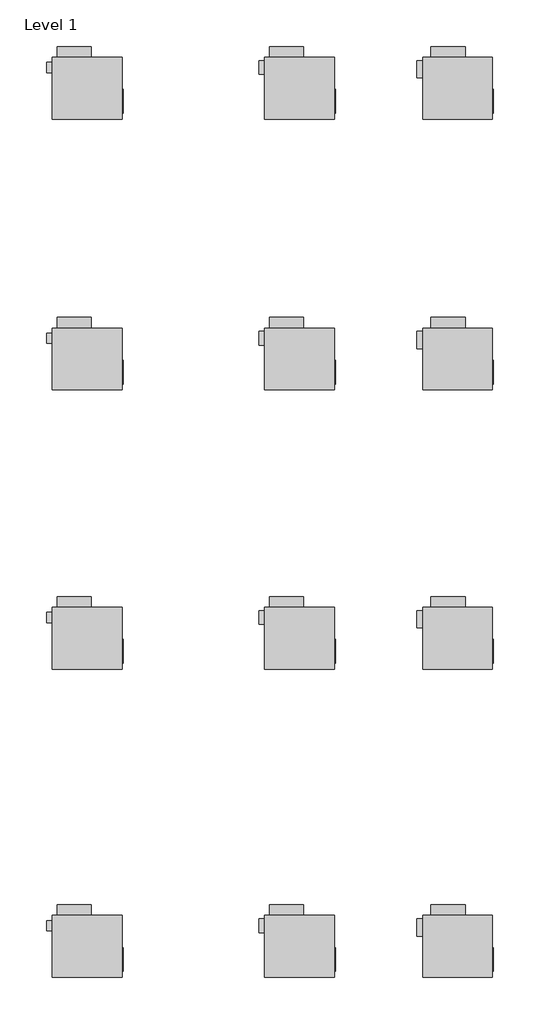
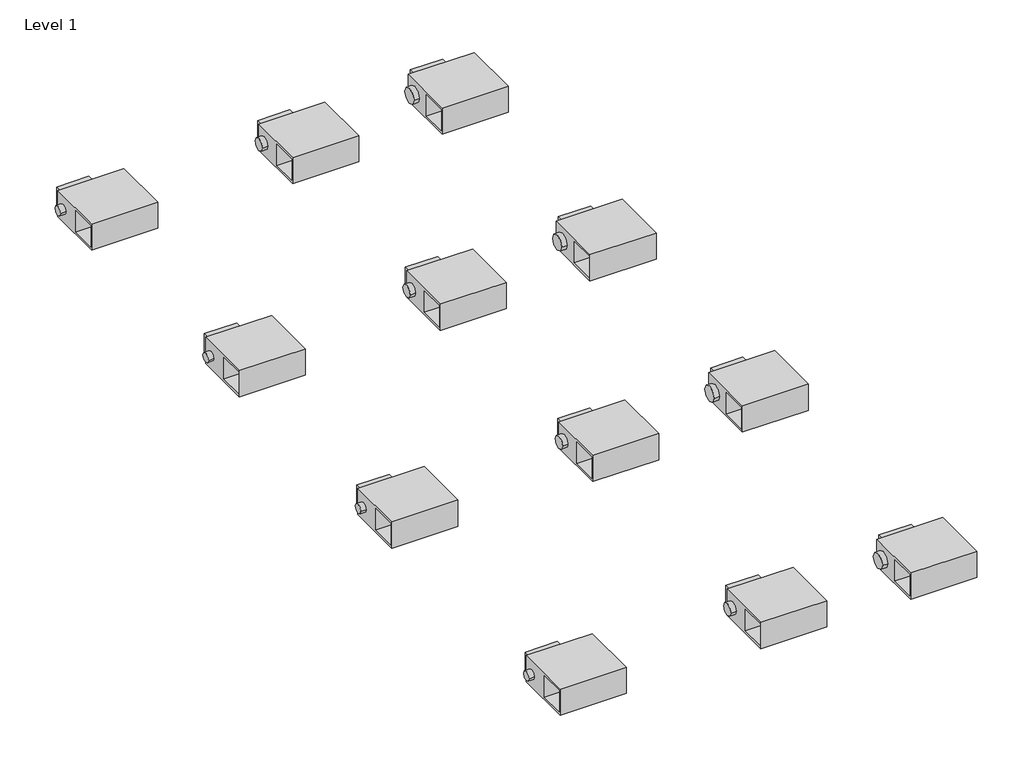
# One storey: 12 proxies.
"""IFC4 building model written with IfcOpenShell, lengths in millimetres."""

import ifcopenshell
import ifcopenshell.guid

model = None  # the IFC model being written
_history = None  # IfcOwnerHistory: only IFC2X3 demands one
_inside = {}  # id of a spatial element -> (the spatial element, [elements in it])
_under = {}  # id of a project, library or spatial element -> (it, [spatial elements below it])
_declared = {}  # id of a project -> (the project, [libraries it declares])
_typed = {}  # id of a type object -> (the type object, [elements of that type])
_made_of = {}  # id of a material, layer set ... -> (it, [elements and type objects made of it])


def new_model(schema):
    """Start an empty IFC model of exactly this schema.

    Asked for "IFC4X3", IfcOpenShell would pick the latest addendum, in which some entities
    have other attributes; the version numbers below select the first issue.
    IFC2X3 requires an IfcOwnerHistory on every rooted entity: one is made here for all.
    """
    global model, _history
    if schema == "IFC4X3":
        model = ifcopenshell.file(schema_version=(4, 3, 0, 0))
    else:
        model = ifcopenshell.file(schema=schema)
    _inside.clear()
    _under.clear()
    _declared.clear()
    _typed.clear()
    _made_of.clear()
    _history = None
    if model.schema == "IFC2X3":
        org = make("IfcOrganization", Name="unknown")
        user = make(
            "IfcPersonAndOrganization",
            ThePerson=make("IfcPerson", FamilyName="unknown"),
            TheOrganization=org,
        )
        app = make(
            "IfcApplication",
            ApplicationDeveloper=org,
            Version="unknown",
            ApplicationFullName="unknown",
            ApplicationIdentifier="unknown",
        )
        _history = make(
            "IfcOwnerHistory",
            OwningUser=user,
            OwningApplication=app,
            ChangeAction="ADDED",
            CreationDate=0,
        )
    return model


def make(cls, **values):
    """One entity of the class cls with the attributes given. An attribute that is None is left unset."""
    return model.create_entity(
        cls, **{name: value for name, value in values.items() if value is not None}
    )


def rooted(cls, **values):
    """An entity with a GlobalId (a new one), such as an element, a storey or a relation."""
    return make(cls, GlobalId=ifcopenshell.guid.new(), OwnerHistory=_history, **values)


def si_unit(unit_type, name, prefix=None):
    """IfcSIUnit, for example si_unit("LENGTHUNIT", "METRE", prefix="MILLI")."""
    return make("IfcSIUnit", UnitType=unit_type, Prefix=prefix, Name=name)


def assignment(units):
    """IfcUnitAssignment: the units of a project."""
    return None if units is None else make("IfcUnitAssignment", Units=units)


def point(xyz):
    """IfcCartesianPoint."""
    return None if xyz is None else make("IfcCartesianPoint", Coordinates=xyz)


def direction(xyz):
    """IfcDirection."""
    return None if xyz is None else make("IfcDirection", DirectionRatios=xyz)


def frame(location, z_axis=None, x_axis=None):
    """IfcAxis2Placement3D, a coordinate frame: its origin and axes. An axis left out is left unset."""
    return make(
        "IfcAxis2Placement3D",
        Location=point(location),
        Axis=direction(z_axis),
        RefDirection=direction(x_axis),
    )


def frame_2d(location, x_axis=None):
    """IfcAxis2Placement2D, a coordinate frame in the plane: its origin and x axis."""
    return make(
        "IfcAxis2Placement2D", Location=point(location), RefDirection=direction(x_axis)
    )


def origin():
    """The frame at (0, 0, 0) with its axes left unset."""
    return frame((0.0, 0.0, 0.0))


def place(relative_to, where):
    """IfcLocalPlacement: puts the frame where relative to a parent placement (None: the world)."""
    return make(
        "IfcLocalPlacement", PlacementRelTo=relative_to, RelativePlacement=where
    )


def context(
    kind, dimensions, precision=None, world=None, true_north=None, identifier=None
):
    """IfcGeometricRepresentationContext, for example the 3D "Model" context."""
    return make(
        "IfcGeometricRepresentationContext",
        ContextIdentifier=identifier,
        ContextType=kind,
        CoordinateSpaceDimension=dimensions,
        Precision=precision,
        WorldCoordinateSystem=world,
        TrueNorth=true_north,
    )


def project(units=None, contexts=None):
    """IfcProject with its units and contexts."""
    return rooted(
        "IfcProject",
        Name="project",
        RepresentationContexts=contexts,
        UnitsInContext=assignment(units),
    )


def spatial(cls, under=None, at=None, **own):
    """A site, building, storey or space (cls), placed at a placement, below another one or the project."""
    s = rooted(cls, ObjectPlacement=at, **own)
    if under is not None:
        _under.setdefault(under.id(), (under, []))[1].append(s)
    return s


def polyline(points):
    """IfcPolyline through the points."""
    return make("IfcPolyline", Points=[point(p) for p in points])


def circle_curve(where, radius):
    """IfcCircle in the frame where."""
    return make("IfcCircle", Position=where, Radius=radius)


def trimmed(basis, trim1, trim2, sense, master):
    """IfcTrimmedCurve: the piece of a basis curve between two trims."""
    return make(
        "IfcTrimmedCurve",
        BasisCurve=basis,
        Trim1=trim1,
        Trim2=trim2,
        SenseAgreement=sense,
        MasterRepresentation=master,
    )


def segment(curve, same_sense, transition):
    """IfcCompositeCurveSegment."""
    return make(
        "IfcCompositeCurveSegment",
        Transition=transition,
        SameSense=same_sense,
        ParentCurve=curve,
    )


def composite_curve(segments, self_intersect=None):
    """IfcCompositeCurve: segments joined end to end."""
    return make("IfcCompositeCurve", Segments=segments, SelfIntersect=self_intersect)


def outline(outer, holes=None, kind="AREA"):
    """IfcArbitraryClosedProfileDef: a profile drawn as a closed curve; with holes, ...WithVoids."""
    if holes is None:
        return make("IfcArbitraryClosedProfileDef", ProfileType=kind, OuterCurve=outer)
    return make(
        "IfcArbitraryProfileDefWithVoids",
        ProfileType=kind,
        OuterCurve=outer,
        InnerCurves=holes,
    )


def extrude(swept, where, along, depth):
    """IfcExtrudedAreaSolid: the profile swept, set in the frame where, extruded along a direction by depth."""
    return make(
        "IfcExtrudedAreaSolid",
        SweptArea=swept,
        Position=where,
        ExtrudedDirection=direction(along),
        Depth=depth,
    )


def faces_of(points, faces, orient=None, outer=None):
    """IfcFace entities. A face is a list of loops; a loop is a list of indices into points, from 0.

    orient and outer hold one flag for each loop. By default every Orientation is true, the
    first loop of a face is its IfcFaceOuterBound and the others are IfcFaceBound.
    """
    made = []
    for i, loops in enumerate(faces):
        bounds = []
        for j, loop in enumerate(loops):
            is_outer = j == 0 if outer is None else outer[i][j]
            bounds.append(
                make(
                    "IfcFaceOuterBound" if is_outer else "IfcFaceBound",
                    Bound=make("IfcPolyLoop", Polygon=[points[k] for k in loop]),
                    Orientation=True if orient is None else orient[i][j],
                )
            )
        made.append(make("IfcFace", Bounds=bounds))
    return made


def faceted_brep(points, faces, orient=None, outer=None, voids=None):
    """IfcFacetedBrep: a solid bounded by flat faces; with voids (closed shells), ...WithVoids."""
    shared = [point(p) for p in points]
    hull = make("IfcClosedShell", CfsFaces=faces_of(shared, faces, orient, outer))
    if voids is None:
        return make("IfcFacetedBrep", Outer=hull)
    return make(
        "IfcFacetedBrepWithVoids",
        Outer=hull,
        Voids=[
            make(cls, CfsFaces=faces_of(shared, fs, o, b)) for cls, fs, o, b in voids
        ],
    )


def shape(context_of_items, identifier, shape_type, items):
    """IfcShapeRepresentation: the items that make up one representation, for example the "Body"."""
    return make(
        "IfcShapeRepresentation",
        ContextOfItems=context_of_items,
        RepresentationIdentifier=identifier,
        RepresentationType=shape_type,
        Items=items,
    )


def source(mapping_origin, context_of_items, identifier, shape_type, items):
    """IfcRepresentationMap: a shape defined once, which mapped items show again and again."""
    return make(
        "IfcRepresentationMap",
        MappingOrigin=mapping_origin,
        MappedRepresentation=shape(context_of_items, identifier, shape_type, items),
    )


def transform(
    local_origin,
    x_axis=None,
    y_axis=None,
    z_axis=None,
    scale=None,
    scale2=None,
    scale3=None,
    uniform=True,
):
    """IfcCartesianTransformationOperator3D, or its non-uniform kind. x_axis, y_axis, z_axis: its Axis1, 2, 3."""
    if uniform:
        return make(
            "IfcCartesianTransformationOperator3D",
            Axis1=direction(x_axis),
            Axis2=direction(y_axis),
            LocalOrigin=point(local_origin),
            Scale=scale,
            Axis3=direction(z_axis),
        )
    return make(
        "IfcCartesianTransformationOperator3DnonUniform",
        Axis1=direction(x_axis),
        Axis2=direction(y_axis),
        LocalOrigin=point(local_origin),
        Scale=scale,
        Axis3=direction(z_axis),
        Scale2=scale2,
        Scale3=scale3,
    )


def mapped(mapping_source, mapping_target):
    """IfcMappedItem: shows the shape of a source again, moved by a transform."""
    return make(
        "IfcMappedItem", MappingSource=mapping_source, MappingTarget=mapping_target
    )


def made_of(thing, what):
    """Note that an element or type object is made of a material, layer set ...; save() writes the relation."""
    if what is not None:
        _made_of.setdefault(what.id(), (what, []))[1].append(thing)
    return thing


def element(
    cls,
    number,
    at=None,
    inside=None,
    cuts=None,
    type_object=None,
    material=None,
    context=None,
    identifier="Body",
    shape_type=None,
    held_by="IfcProductDefinitionShape",
    body=None,
    shapes=None,
    **own,
):
    """One element of the class cls, such as IfcWall. Its Tag is "e" and its number.

    at: its placement. inside: the storey or other place that contains it. cuts: it is an
    opening in that element (IfcRelVoidsElement). A single representation is given by context,
    identifier, shape_type and body (its items); several are given by shapes. held_by: the class
    of the entity that holds the representations. save() writes the other relations.
    """
    e = rooted(cls, Tag="e%d" % number, ObjectPlacement=at, **own)
    if body is not None:
        shapes = [shape(context, identifier, shape_type, body)]
    if shapes is not None:
        e.Representation = make(held_by, Representations=shapes)
    if inside is not None:
        _inside.setdefault(inside.id(), (inside, []))[1].append(e)
    if cuts is not None:
        rooted(
            "IfcRelVoidsElement", RelatingBuildingElement=cuts, RelatedOpeningElement=e
        )
    if type_object is not None:
        _typed.setdefault(type_object.id(), (type_object, []))[1].append(e)
    return made_of(e, material)


def aggregate(whole, parts):
    """IfcRelAggregates: a whole, such as a stair, and the parts it consists of."""
    return rooted("IfcRelAggregates", RelatingObject=whole, RelatedObjects=parts)


def save(model, path):
    """Write the relations noted so far, then the file.

    IfcRelAggregates (storeys below a building ...), IfcRelContainedInSpatialStructure (elements
    in a storey), IfcRelDefinesByType, IfcRelAssociatesMaterial and IfcRelDeclares: one each for
    every whole, place, type object, material and project.
    """
    for whole, parts in _under.values():
        aggregate(whole, parts)
    for where, things in _inside.values():
        rooted(
            "IfcRelContainedInSpatialStructure",
            RelatedElements=things,
            RelatingStructure=where,
        )
    for kind, things in _typed.values():
        rooted("IfcRelDefinesByType", RelatedObjects=things, RelatingType=kind)
    for what, things in _made_of.values():
        rooted("IfcRelAssociatesMaterial", RelatedObjects=things, RelatingMaterial=what)
    for by, libraries in _declared.values():
        rooted("IfcRelDeclares", RelatingContext=by, RelatedDefinitions=libraries)
    model.write(path)


def vav_unit_parallel_fan_powered_size_2_10_inch_inlet_b65b1531(model_context):
    return source(origin(), model_context, "Body", "SolidModel", [
        extrude(outline(polyline([(531.8125, -15.875), (531.8125, -371.475), (519.1125, -371.475), (519.1125, -15.875), (531.8125, -15.875)])), frame((0.0, 0.0, -139.7), z_axis=(0.0, 0.0, 1.0), x_axis=(1.0, 0.0, 0.0)), (0.0, 0.0, 1.0), 279.4),
        extrude(outline(polyline([(112.7125, 460.375), (-395.2875, 460.375), (-395.2875, 619.125), (112.7125, 619.125), (112.7125, 460.375)])), frame((0.0, 0.0, -152.4), z_axis=(0.0, 0.0, 1.0), x_axis=(1.0, 0.0, 0.0)), (0.0, 0.0, 1.0), 304.8),
        extrude(outline(composite_curve([segment(trimmed(circle_curve(frame_2d((282.575, 0.0)), 127.0), [point((155.575, 0.0))], [point((409.575, 0.0))], False, "CARTESIAN"), True, "CONTINUOUS"), segment(trimmed(circle_curve(frame_2d((282.575, 0.0)), 127.0), [point((409.575, 0.0))], [point((155.575, 0.0))], False, "CARTESIAN"), True, "CONTINUOUS")], self_intersect=False)), frame((-604.8375, 0.0, 0.0), z_axis=(1.0, 0.0, 0.0), x_axis=(0.0, 1.0, 0.0)), (0.0, 0.0, 1.0), 85.725),
        faceted_brep([(519.1125, 460.375, 217.4875), (-519.1125, 460.375, 217.4875), (-519.1125, -460.375, 217.4875), (519.1125, -460.375, 217.4875), (519.1125, 460.375, -217.4875), (519.1125, -460.375, -217.4875), (-519.1125, -460.375, -217.4875), (-519.1125, 460.375, -217.4875), (-519.1125, -434.975, 177.8), (-519.1125, -434.975, -177.8), (-519.1125, -28.575, -177.8), (-519.1125, -28.575, 177.8), (0.0, -434.975, 177.8), (0.0, -28.575, 177.8), (0.0, -28.575, -177.8), (0.0, -434.975, -177.8)], [[[0, 1, 2, 3]], [[4, 5, 6, 7]], [[1, 0, 4, 7]], [[2, 1, 7, 6], [8, 9, 10, 11]], [[3, 2, 6, 5]], [[0, 3, 5, 4]], [[12, 13, 14, 15]], [[12, 15, 9, 8]], [[15, 14, 10, 9]], [[14, 13, 11, 10]], [[13, 12, 8, 11]]]),
    ])


def vav_unit_parallel_fan_powered_size_2_6_inch_inlet_6222e6d5(model_context):
    return source(origin(), model_context, "Body", "SolidModel", [
        extrude(outline(polyline([(531.8125, -15.875), (531.8125, -371.475), (519.1125, -371.475), (519.1125, -15.875), (531.8125, -15.875)])), frame((0.0, 0.0, -139.7), z_axis=(0.0, 0.0, 1.0), x_axis=(1.0, 0.0, 0.0)), (0.0, 0.0, 1.0), 279.4),
        extrude(outline(polyline([(61.9125, 460.375), (-446.0875, 460.375), (-446.0875, 619.125), (61.9125, 619.125), (61.9125, 460.375)])), frame((0.0, 0.0, -152.4), z_axis=(0.0, 0.0, 1.0), x_axis=(1.0, 0.0, 0.0)), (0.0, 0.0, 1.0), 304.8),
        extrude(outline(composite_curve([segment(trimmed(circle_curve(frame_2d((307.975, 0.0)), 76.2), [point((231.775, 0.0))], [point((384.175, 0.0))], False, "CARTESIAN"), True, "CONTINUOUS"), segment(trimmed(circle_curve(frame_2d((307.975, 0.0)), 76.2), [point((384.175, 0.0))], [point((231.775, 0.0))], False, "CARTESIAN"), True, "CONTINUOUS")], self_intersect=False)), frame((-604.8375, 0.0, 0.0), z_axis=(1.0, 0.0, 0.0), x_axis=(0.0, 1.0, 0.0)), (0.0, 0.0, 1.0), 85.725),
        faceted_brep([(519.1125, 460.375, 217.4875), (-519.1125, 460.375, 217.4875), (-519.1125, -460.375, 217.4875), (519.1125, -460.375, 217.4875), (519.1125, 460.375, -217.4875), (519.1125, -460.375, -217.4875), (-519.1125, -460.375, -217.4875), (-519.1125, 460.375, -217.4875), (-519.1125, -434.975, 177.8), (-519.1125, -434.975, -177.8), (-519.1125, -28.575, -177.8), (-519.1125, -28.575, 177.8), (0.0, -434.975, 177.8), (0.0, -28.575, 177.8), (0.0, -28.575, -177.8), (0.0, -434.975, -177.8)], [[[0, 1, 2, 3]], [[4, 5, 6, 7]], [[1, 0, 4, 7]], [[2, 1, 7, 6], [8, 9, 10, 11]], [[3, 2, 6, 5]], [[0, 3, 5, 4]], [[12, 13, 14, 15]], [[12, 15, 9, 8]], [[15, 14, 10, 9]], [[14, 13, 11, 10]], [[13, 12, 8, 11]]]),
    ])


def vav_unit_parallel_fan_powered_size_2_8_inch_inlet_1779b90c(model_context):
    return source(origin(), model_context, "Body", "SolidModel", [
        extrude(outline(polyline([(531.8125, -15.875), (531.8125, -371.475), (519.1125, -371.475), (519.1125, -15.875), (531.8125, -15.875)])), frame((0.0, 0.0, -139.7), z_axis=(0.0, 0.0, 1.0), x_axis=(1.0, 0.0, 0.0)), (0.0, 0.0, 1.0), 279.4),
        extrude(outline(polyline([(61.9125, 460.375), (-446.0875, 460.375), (-446.0875, 619.125), (61.9125, 619.125), (61.9125, 460.375)])), frame((0.0, 0.0, -152.4), z_axis=(0.0, 0.0, 1.0), x_axis=(1.0, 0.0, 0.0)), (0.0, 0.0, 1.0), 304.8),
        extrude(outline(composite_curve([segment(trimmed(circle_curve(frame_2d((307.975, 0.0)), 101.6), [point((206.375, 0.0))], [point((409.575, 0.0))], False, "CARTESIAN"), True, "CONTINUOUS"), segment(trimmed(circle_curve(frame_2d((307.975, 0.0)), 101.6), [point((409.575, 0.0))], [point((206.375, 0.0))], False, "CARTESIAN"), True, "CONTINUOUS")], self_intersect=False)), frame((-604.8375, 0.0, 0.0), z_axis=(1.0, 0.0, 0.0), x_axis=(0.0, 1.0, 0.0)), (0.0, 0.0, 1.0), 85.725),
        faceted_brep([(519.1125, 460.375, 217.4875), (-519.1125, 460.375, 217.4875), (-519.1125, -460.375, 217.4875), (519.1125, -460.375, 217.4875), (519.1125, 460.375, -217.4875), (519.1125, -460.375, -217.4875), (-519.1125, -460.375, -217.4875), (-519.1125, 460.375, -217.4875), (-519.1125, -434.975, 177.8), (-519.1125, -434.975, -177.8), (-519.1125, -28.575, -177.8), (-519.1125, -28.575, 177.8), (0.0, -434.975, 177.8), (0.0, -28.575, 177.8), (0.0, -28.575, -177.8), (0.0, -434.975, -177.8)], [[[0, 1, 2, 3]], [[4, 5, 6, 7]], [[1, 0, 4, 7]], [[2, 1, 7, 6], [8, 9, 10, 11]], [[3, 2, 6, 5]], [[0, 3, 5, 4]], [[12, 13, 14, 15]], [[12, 15, 9, 8]], [[15, 14, 10, 9]], [[14, 13, 11, 10]], [[13, 12, 8, 11]]]),
    ])


model = new_model("IFC4")

# Units and contexts
model_context = context("Model", 3, world=origin())
ifc_project = project(units=[si_unit("LENGTHUNIT", "METRE", prefix="MILLI")], contexts=[model_context])

# Site, building, storey
site = spatial("IfcSite", under=ifc_project)
building = spatial("IfcBuilding", under=site)
storey = spatial("IfcBuildingStorey", under=building, Name="Level 1", Elevation=0.0)

# Proxies
placement = place(None, origin())
vav_unit_parallel_fan_powered_size_2_10_inch_inlet_shape = vav_unit_parallel_fan_powered_size_2_10_inch_inlet_b65b1531(model_context)
element("IfcBuildingElementProxy", 1, Name="VAV Unit - Parallel Fan Powered : Size 2 - 10 inch Inlet", ObjectType="VAV Unit - Parallel Fan Powered : Size 2 - 10 inch Inlet", at=placement, inside=storey, context=model_context, shape_type="MappedRepresentation", body=[
    mapped(vav_unit_parallel_fan_powered_size_2_10_inch_inlet_shape, transform((-7137.4442191, 12797.9424061, 0.0), x_axis=(1.0, 0.0, 0.0), y_axis=(0.0, 1.0, 0.0), z_axis=(0.0, 0.0, 1.0))),
])
element("IfcBuildingElementProxy", 2, Name="VAV Unit - Parallel Fan Powered : Size 2 - 10 inch Inlet", ObjectType="VAV Unit - Parallel Fan Powered : Size 2 - 10 inch Inlet", at=placement, inside=storey, context=model_context, shape_type="MappedRepresentation", body=[
    mapped(vav_unit_parallel_fan_powered_size_2_10_inch_inlet_shape, transform((-7137.4442191, 8773.2773935, 0.0), x_axis=(1.0, 0.0, 0.0), y_axis=(0.0, 1.0, 0.0), z_axis=(0.0, 0.0, 1.0))),
])
element("IfcBuildingElementProxy", 3, Name="VAV Unit - Parallel Fan Powered : Size 2 - 10 inch Inlet", ObjectType="VAV Unit - Parallel Fan Powered : Size 2 - 10 inch Inlet", at=placement, inside=storey, context=model_context, shape_type="MappedRepresentation", body=[
    mapped(vav_unit_parallel_fan_powered_size_2_10_inch_inlet_shape, transform((-7137.4442191, 4624.7765344, 0.0), x_axis=(1.0, 0.0, 0.0), y_axis=(0.0, 1.0, 0.0), z_axis=(0.0, 0.0, 1.0))),
])
element("IfcBuildingElementProxy", 4, Name="VAV Unit - Parallel Fan Powered : Size 2 - 10 inch Inlet", ObjectType="VAV Unit - Parallel Fan Powered : Size 2 - 10 inch Inlet", at=placement, inside=storey, context=model_context, shape_type="MappedRepresentation", body=[
    mapped(vav_unit_parallel_fan_powered_size_2_10_inch_inlet_shape, transform((-7137.4442191, 42.8502123, 0.0), x_axis=(1.0, 0.0, 0.0), y_axis=(0.0, 1.0, 0.0), z_axis=(0.0, 0.0, 1.0))),
])
vav_unit_parallel_fan_powered_size_2_6_inch_inlet_shape = vav_unit_parallel_fan_powered_size_2_6_inch_inlet_6222e6d5(model_context)
element("IfcBuildingElementProxy", 5, Name="VAV Unit - Parallel Fan Powered : Size 2 - 6 inch Inlet", ObjectType="VAV Unit - Parallel Fan Powered : Size 2 - 6 inch Inlet", at=placement, inside=storey, context=model_context, shape_type="MappedRepresentation", body=[
    mapped(vav_unit_parallel_fan_powered_size_2_6_inch_inlet_shape, transform((-12648.1393902, 12797.9424061, 0.0), x_axis=(1.0, 0.0, 0.0), y_axis=(0.0, 1.0, 0.0), z_axis=(0.0, 0.0, 1.0))),
])
element("IfcBuildingElementProxy", 6, Name="VAV Unit - Parallel Fan Powered : Size 2 - 6 inch Inlet", ObjectType="VAV Unit - Parallel Fan Powered : Size 2 - 6 inch Inlet", at=placement, inside=storey, context=model_context, shape_type="MappedRepresentation", body=[
    mapped(vav_unit_parallel_fan_powered_size_2_6_inch_inlet_shape, transform((-12648.1393902, 8773.2773935, 0.0), x_axis=(1.0, 0.0, 0.0), y_axis=(0.0, 1.0, 0.0), z_axis=(0.0, 0.0, 1.0))),
])
element("IfcBuildingElementProxy", 7, Name="VAV Unit - Parallel Fan Powered : Size 2 - 6 inch Inlet", ObjectType="VAV Unit - Parallel Fan Powered : Size 2 - 6 inch Inlet", at=placement, inside=storey, context=model_context, shape_type="MappedRepresentation", body=[
    mapped(vav_unit_parallel_fan_powered_size_2_6_inch_inlet_shape, transform((-12648.1393902, 4624.7765344, 0.0), x_axis=(1.0, 0.0, 0.0), y_axis=(0.0, 1.0, 0.0), z_axis=(0.0, 0.0, 1.0))),
])
element("IfcBuildingElementProxy", 8, Name="VAV Unit - Parallel Fan Powered : Size 2 - 6 inch Inlet", ObjectType="VAV Unit - Parallel Fan Powered : Size 2 - 6 inch Inlet", at=placement, inside=storey, context=model_context, shape_type="MappedRepresentation", body=[
    mapped(vav_unit_parallel_fan_powered_size_2_6_inch_inlet_shape, transform((-12648.1393902, 42.8502123, 0.0), x_axis=(1.0, 0.0, 0.0), y_axis=(0.0, 1.0, 0.0), z_axis=(0.0, 0.0, 1.0))),
])
vav_unit_parallel_fan_powered_size_2_8_inch_inlet_shape = vav_unit_parallel_fan_powered_size_2_8_inch_inlet_1779b90c(model_context)
element("IfcBuildingElementProxy", 9, Name="VAV Unit - Parallel Fan Powered : Size 2 - 8 inch Inlet", ObjectType="VAV Unit - Parallel Fan Powered : Size 2 - 8 inch Inlet", at=placement, inside=storey, context=model_context, shape_type="MappedRepresentation", body=[
    mapped(vav_unit_parallel_fan_powered_size_2_8_inch_inlet_shape, transform((-9490.3253034, 12797.9424061, 0.0), x_axis=(1.0, 0.0, 0.0), y_axis=(0.0, 1.0, 0.0), z_axis=(0.0, 0.0, 1.0))),
])
element("IfcBuildingElementProxy", 10, Name="VAV Unit - Parallel Fan Powered : Size 2 - 8 inch Inlet", ObjectType="VAV Unit - Parallel Fan Powered : Size 2 - 8 inch Inlet", at=placement, inside=storey, context=model_context, shape_type="MappedRepresentation", body=[
    mapped(vav_unit_parallel_fan_powered_size_2_8_inch_inlet_shape, transform((-9490.3253034, 8773.2773935, 0.0), x_axis=(1.0, 0.0, 0.0), y_axis=(0.0, 1.0, 0.0), z_axis=(0.0, 0.0, 1.0))),
])
element("IfcBuildingElementProxy", 11, Name="VAV Unit - Parallel Fan Powered : Size 2 - 8 inch Inlet", ObjectType="VAV Unit - Parallel Fan Powered : Size 2 - 8 inch Inlet", at=placement, inside=storey, context=model_context, shape_type="MappedRepresentation", body=[
    mapped(vav_unit_parallel_fan_powered_size_2_8_inch_inlet_shape, transform((-9490.3253034, 4624.7765344, 0.0), x_axis=(1.0, 0.0, 0.0), y_axis=(0.0, 1.0, 0.0), z_axis=(0.0, 0.0, 1.0))),
])
element("IfcBuildingElementProxy", 12, Name="VAV Unit - Parallel Fan Powered : Size 2 - 8 inch Inlet", ObjectType="VAV Unit - Parallel Fan Powered : Size 2 - 8 inch Inlet", at=placement, inside=storey, context=model_context, shape_type="MappedRepresentation", body=[
    mapped(vav_unit_parallel_fan_powered_size_2_8_inch_inlet_shape, transform((-9490.3253034, 42.8502123, 0.0), x_axis=(1.0, 0.0, 0.0), y_axis=(0.0, 1.0, 0.0), z_axis=(0.0, 0.0, 1.0))),
])

save(model, "model.ifc")

# Revit data of these elements
# Project information
#   Project Issue Date = "Issue Date"
#   Project Status = "Project Status"
#   Client Name = "Owner"
#   Project Address = "Enter address here"
#   Project Name = "Project Name"
#   Project Number = "Project Number"
# Type "VAV Unit - Parallel Fan Powered : Size 2 - 10 inch Inlet"
#   Width2 = 1' - 2"
#   Voltage = 120 V
#   UnitWidth = 3' - 4 7/8"
#   UnitHeight = 3' - 0 1/4"
#   UnitDepth = 1' - 5 1/8"
#   SupplyConnectorWidth = 1' - 2"
#   SupplyConnectorVerticalOffset = 0' - 2 1/8"
#   SupplyConnectorLength = 0' - 0 1/2"
#   SupplyConnectorHorizontalOffset = 0' - 3 1/2"
#   SupplyConnectorDepth = 0' - 11"
#   SupplyAirConnectorCenterOffset = 0' - 10 1/2"
#   PrimaryToSupplyRatio [instance default] = 0.2
#   PrimaryAirOffset = 0' - 7"
#   PrimaryAirFlow [instance default] = 280 CFM
#   PrimaryAirConnectorVerticalOffset = 0' - 8 9/16"
#   PrimaryAirConnectorRadius = 0' - 5"
#   PrimaryAirConnectorLength = 0' - 3 3/8"
#   PrimaryAirConnectorDiameter = 0' - 10"
#   PrimaryAirConnectorCenterOffset = 0' - 7"
#   Pressure Drop [instance default] = 0.01 in-wg
#   InducedAirInletWidth = 1' - 4"
#   InducedAirInletDepth = 1' - 2"
#   InducedAirConnectorHorizontalOffset = 0' - 1"
#   InducedAirConnectorCenterOffset = 0' - 9"
#   Height2 = 0' - 11"
#   ElectricalConnectionBoxWidth = 1' - 8"
#   ElectricalConnectionBoxOffset = 0' - 4 7/8"
#   ElectricalConnectionBoxHeight = 0' - 6 1/4"
#   ElectricalConnectionBoxDepth = 1' - 0"
#   SupplyAirFlow [instance default] = 1400 CFM
#   Apparent Load = 542 VA
#   SupplyAirConnectorIndex = 2
#   PrimaryAirConnectorIndex = 1
#   Number of Poles = 1
#   InducedAirConnectorIndex = 3
#   VAV Material = none
#   Load Classification = Cooling
#   Default Elevation = 0
#   Assembly Code = ""
# Type "VAV Unit - Parallel Fan Powered : Size 2 - 6 inch Inlet"
#   Width2 = 1' - 2"
#   Voltage = 120 V
#   UnitWidth = 3' - 4 7/8"
#   UnitHeight = 3' - 0 1/4"
#   UnitDepth = 1' - 5 1/8"
#   SupplyConnectorWidth = 1' - 2"
#   SupplyConnectorVerticalOffset = 0' - 2 1/8"
#   SupplyConnectorLength = 0' - 0 1/2"
#   SupplyConnectorHorizontalOffset = 0' - 3 1/2"
#   SupplyConnectorDepth = 0' - 11"
#   SupplyAirConnectorCenterOffset = 0' - 10 1/2"
#   PrimaryToSupplyRatio [instance default] = 0.2
#   PrimaryAirOffset = 0' - 6"
#   PrimaryAirFlow [instance default] = 100 CFM
#   PrimaryAirConnectorVerticalOffset = 0' - 8 9/16"
#   PrimaryAirConnectorRadius = 0' - 3"
#   PrimaryAirConnectorLength = 0' - 3 3/8"
#   PrimaryAirConnectorDiameter = 0' - 6"
#   PrimaryAirConnectorCenterOffset = 0' - 6"
#   Pressure Drop [instance default] = 0.04 in-wg
#   InducedAirInletWidth = 1' - 4"
#   InducedAirInletDepth = 1' - 2"
#   InducedAirConnectorHorizontalOffset = 0' - 1"
#   InducedAirConnectorCenterOffset = 0' - 9"
#   Height2 = 0' - 11"
#   ElectricalConnectionBoxWidth = 1' - 8"
#   ElectricalConnectionBoxOffset = 0' - 2 7/8"
#   ElectricalConnectionBoxHeight = 0' - 6 1/4"
#   ElectricalConnectionBoxDepth = 1' - 0"
#   SupplyAirFlow [instance default] = 500 CFM
#   Apparent Load = 181 VA
#   SupplyAirConnectorIndex = 2
#   PrimaryAirConnectorIndex = 1
#   Number of Poles = 1
#   InducedAirConnectorIndex = 3
#   VAV Material = none
#   Load Classification = Cooling
#   Default Elevation = 0
#   Assembly Code = ""
# Type "VAV Unit - Parallel Fan Powered : Size 2 - 8 inch Inlet"
#   Width2 = 1' - 2"
#   Voltage = 120 V
#   UnitWidth = 3' - 4 7/8"
#   UnitHeight = 3' - 0 1/4"
#   UnitDepth = 1' - 5 1/8"
#   SupplyConnectorWidth = 1' - 2"
#   SupplyConnectorVerticalOffset = 0' - 2 1/8"
#   SupplyConnectorLength = 0' - 0 1/2"
#   SupplyConnectorHorizontalOffset = 0' - 3 1/2"
#   SupplyConnectorDepth = 0' - 11"
#   SupplyAirConnectorCenterOffset = 0' - 10 1/2"
#   PrimaryToSupplyRatio [instance default] = 0.2
#   PrimaryAirOffset = 0' - 6"
#   PrimaryAirFlow [instance default] = 180 CFM
#   PrimaryAirConnectorVerticalOffset = 0' - 8 9/16"
#   PrimaryAirConnectorRadius = 0' - 4"
#   PrimaryAirConnectorLength = 0' - 3 3/8"
#   PrimaryAirConnectorDiameter = 0' - 8"
#   PrimaryAirConnectorCenterOffset = 0' - 6"
#   Pressure Drop [instance default] = 0.02 in-wg
#   InducedAirInletWidth = 1' - 4"
#   InducedAirInletDepth = 1' - 2"
#   InducedAirConnectorHorizontalOffset = 0' - 1"
#   InducedAirConnectorCenterOffset = 0' - 9"
#   Height2 = 0' - 11"
#   ElectricalConnectionBoxWidth = 1' - 8"
#   ElectricalConnectionBoxOffset = 0' - 2 7/8"
#   ElectricalConnectionBoxHeight = 0' - 6 1/4"
#   ElectricalConnectionBoxDepth = 1' - 0"
#   SupplyAirFlow [instance default] = 900 CFM
#   Apparent Load = 271 VA
#   SupplyAirConnectorIndex = 2
#   PrimaryAirConnectorIndex = 1
#   Number of Poles = 1
#   InducedAirConnectorIndex = 3
#   VAV Material = none
#   Load Classification = Cooling
#   Default Elevation = 0
#   Assembly Code = ""
# Element 1 (IfcBuildingElementProxy, "VAV Unit - Parallel Fan Powered : Size 2 - 10 inch Inlet")
#   Mark = "9"
#   SupplyAirFlow = 1400 CFM
#   PrimaryToSupplyRatio = 0.2
#   PrimaryAirFlow = 280 CFM
#   Pressure Drop = 0.01 in-wg
#   Phase Created = New Construction
# Element 2 (IfcBuildingElementProxy, "VAV Unit - Parallel Fan Powered : Size 2 - 10 inch Inlet")
#   Mark = "10"
#   SupplyAirFlow = 1400 CFM
#   PrimaryToSupplyRatio = 0.2
#   PrimaryAirFlow = 280 CFM
#   Pressure Drop = 0.01 in-wg
#   Phase Created = New Construction
# Element 3 (IfcBuildingElementProxy, "VAV Unit - Parallel Fan Powered : Size 2 - 10 inch Inlet")
#   Mark = "11"
#   SupplyAirFlow = 1400 CFM
#   PrimaryToSupplyRatio = 0.2
#   PrimaryAirFlow = 280 CFM
#   Pressure Drop = 0.01 in-wg
#   Phase Created = New Construction
# Element 4 (IfcBuildingElementProxy, "VAV Unit - Parallel Fan Powered : Size 2 - 10 inch Inlet")
#   Mark = "12"
#   SupplyAirFlow = 1400 CFM
#   PrimaryToSupplyRatio = 0.2
#   PrimaryAirFlow = 280 CFM
#   Pressure Drop = 0.01 in-wg
#   Phase Created = New Construction
# Element 5 (IfcBuildingElementProxy, "VAV Unit - Parallel Fan Powered : Size 2 - 6 inch Inlet")
#   Mark = "1"
#   SupplyAirFlow = 500 CFM
#   PrimaryToSupplyRatio = 0.2
#   PrimaryAirFlow = 100 CFM
#   Pressure Drop = 0.04 in-wg
#   Phase Created = New Construction
# Element 6 (IfcBuildingElementProxy, "VAV Unit - Parallel Fan Powered : Size 2 - 6 inch Inlet")
#   Mark = "2"
#   SupplyAirFlow = 500 CFM
#   PrimaryToSupplyRatio = 0.2
#   PrimaryAirFlow = 100 CFM
#   Pressure Drop = 0.04 in-wg
#   Phase Created = New Construction
# Element 7 (IfcBuildingElementProxy, "VAV Unit - Parallel Fan Powered : Size 2 - 6 inch Inlet")
#   Mark = "3"
#   SupplyAirFlow = 500 CFM
#   PrimaryToSupplyRatio = 0.2
#   PrimaryAirFlow = 100 CFM
#   Pressure Drop = 0.04 in-wg
#   Phase Created = New Construction
# Element 8 (IfcBuildingElementProxy, "VAV Unit - Parallel Fan Powered : Size 2 - 6 inch Inlet")
#   Mark = "4"
#   SupplyAirFlow = 500 CFM
#   PrimaryToSupplyRatio = 0.2
#   PrimaryAirFlow = 100 CFM
#   Pressure Drop = 0.04 in-wg
#   Phase Created = New Construction
# Element 9 (IfcBuildingElementProxy, "VAV Unit - Parallel Fan Powered : Size 2 - 8 inch Inlet")
#   Mark = "5"
#   SupplyAirFlow = 900 CFM
#   PrimaryToSupplyRatio = 0.2
#   PrimaryAirFlow = 180 CFM
#   Pressure Drop = 0.02 in-wg
#   Phase Created = New Construction
# Element 10 (IfcBuildingElementProxy, "VAV Unit - Parallel Fan Powered : Size 2 - 8 inch Inlet")
#   Mark = "6"
#   SupplyAirFlow = 900 CFM
#   PrimaryToSupplyRatio = 0.2
#   PrimaryAirFlow = 180 CFM
#   Pressure Drop = 0.02 in-wg
#   Phase Created = New Construction
# Element 11 (IfcBuildingElementProxy, "VAV Unit - Parallel Fan Powered : Size 2 - 8 inch Inlet")
#   Mark = "7"
#   SupplyAirFlow = 900 CFM
#   PrimaryToSupplyRatio = 0.2
#   PrimaryAirFlow = 180 CFM
#   Pressure Drop = 0.02 in-wg
#   Phase Created = New Construction
# Element 12 (IfcBuildingElementProxy, "VAV Unit - Parallel Fan Powered : Size 2 - 8 inch Inlet")
#   Mark = "8"
#   SupplyAirFlow = 900 CFM
#   PrimaryToSupplyRatio = 0.2
#   PrimaryAirFlow = 180 CFM
#   Pressure Drop = 0.02 in-wg
#   Phase Created = New Construction
